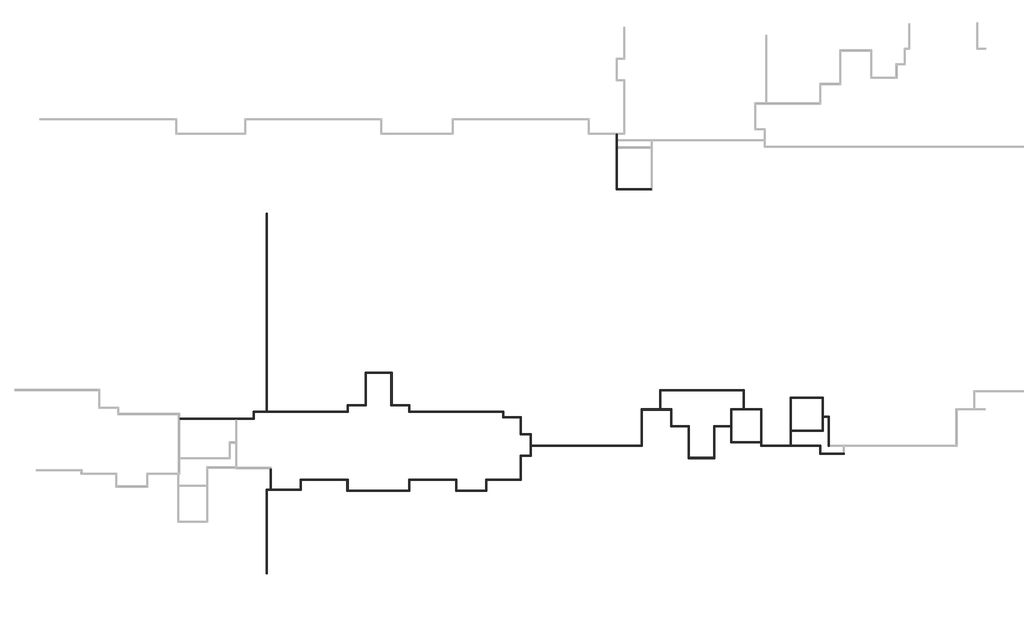
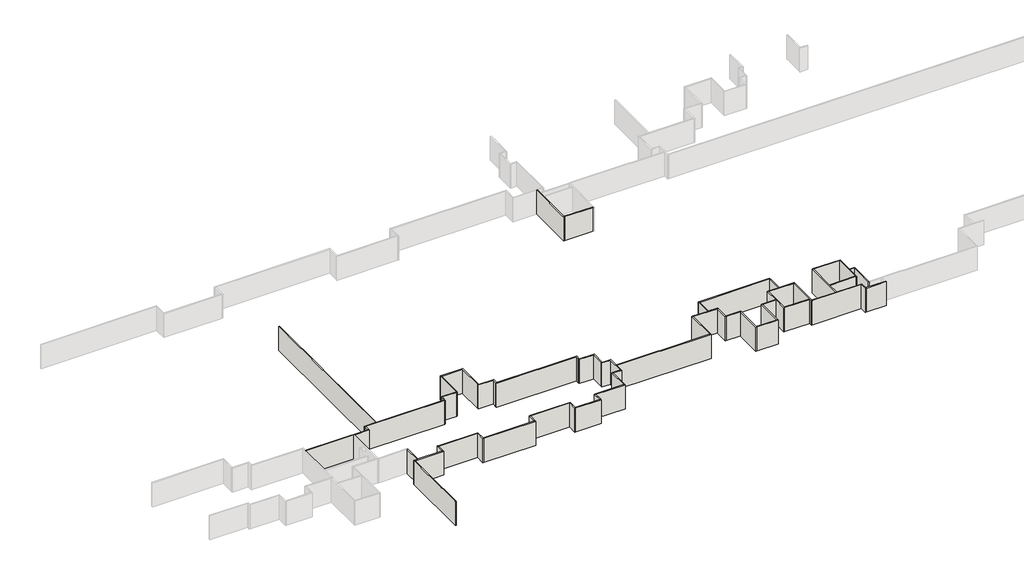
# One storey, part 4 of 8: 59 walls.
"""IFC4 building model written with IfcOpenShell, lengths in millimetres."""

import ifcopenshell
import ifcopenshell.guid

model = None  # the IFC model being written
_history = None  # IfcOwnerHistory: only IFC2X3 demands one
_inside = {}  # id of a spatial element -> (the spatial element, [elements in it])
_under = {}  # id of a project, library or spatial element -> (it, [spatial elements below it])
_declared = {}  # id of a project -> (the project, [libraries it declares])
_typed = {}  # id of a type object -> (the type object, [elements of that type])
_made_of = {}  # id of a material, layer set ... -> (it, [elements and type objects made of it])


def new_model(schema):
    """Start an empty IFC model of exactly this schema.

    Asked for "IFC4X3", IfcOpenShell would pick the latest addendum, in which some entities
    have other attributes; the version numbers below select the first issue.
    IFC2X3 requires an IfcOwnerHistory on every rooted entity: one is made here for all.
    """
    global model, _history
    if schema == "IFC4X3":
        model = ifcopenshell.file(schema_version=(4, 3, 0, 0))
    else:
        model = ifcopenshell.file(schema=schema)
    _inside.clear()
    _under.clear()
    _declared.clear()
    _typed.clear()
    _made_of.clear()
    _history = None
    if model.schema == "IFC2X3":
        org = make("IfcOrganization", Name="unknown")
        user = make(
            "IfcPersonAndOrganization",
            ThePerson=make("IfcPerson", FamilyName="unknown"),
            TheOrganization=org,
        )
        app = make(
            "IfcApplication",
            ApplicationDeveloper=org,
            Version="unknown",
            ApplicationFullName="unknown",
            ApplicationIdentifier="unknown",
        )
        _history = make(
            "IfcOwnerHistory",
            OwningUser=user,
            OwningApplication=app,
            ChangeAction="ADDED",
            CreationDate=0,
        )
    return model


def make(cls, **values):
    """One entity of the class cls with the attributes given. An attribute that is None is left unset."""
    return model.create_entity(
        cls, **{name: value for name, value in values.items() if value is not None}
    )


def rooted(cls, **values):
    """An entity with a GlobalId (a new one), such as an element, a storey or a relation."""
    return make(cls, GlobalId=ifcopenshell.guid.new(), OwnerHistory=_history, **values)


def si_unit(unit_type, name, prefix=None):
    """IfcSIUnit, for example si_unit("LENGTHUNIT", "METRE", prefix="MILLI")."""
    return make("IfcSIUnit", UnitType=unit_type, Prefix=prefix, Name=name)


def assignment(units):
    """IfcUnitAssignment: the units of a project."""
    return None if units is None else make("IfcUnitAssignment", Units=units)


def point(xyz):
    """IfcCartesianPoint."""
    return None if xyz is None else make("IfcCartesianPoint", Coordinates=xyz)


def direction(xyz):
    """IfcDirection."""
    return None if xyz is None else make("IfcDirection", DirectionRatios=xyz)


def frame(location, z_axis=None, x_axis=None):
    """IfcAxis2Placement3D, a coordinate frame: its origin and axes. An axis left out is left unset."""
    return make(
        "IfcAxis2Placement3D",
        Location=point(location),
        Axis=direction(z_axis),
        RefDirection=direction(x_axis),
    )


def origin():
    """The frame at (0, 0, 0) with its axes left unset."""
    return frame((0.0, 0.0, 0.0))


def origin_with_axes():
    """The frame at (0, 0, 0) with the z axis (0, 0, 1) and the x axis (1, 0, 0) written out."""
    return frame((0.0, 0.0, 0.0), z_axis=(0.0, 0.0, 1.0), x_axis=(1.0, 0.0, 0.0))


def place(relative_to, where):
    """IfcLocalPlacement: puts the frame where relative to a parent placement (None: the world)."""
    return make(
        "IfcLocalPlacement", PlacementRelTo=relative_to, RelativePlacement=where
    )


def context(
    kind, dimensions, precision=None, world=None, true_north=None, identifier=None
):
    """IfcGeometricRepresentationContext, for example the 3D "Model" context."""
    return make(
        "IfcGeometricRepresentationContext",
        ContextIdentifier=identifier,
        ContextType=kind,
        CoordinateSpaceDimension=dimensions,
        Precision=precision,
        WorldCoordinateSystem=world,
        TrueNorth=true_north,
    )


def project(units=None, contexts=None):
    """IfcProject with its units and contexts."""
    return rooted(
        "IfcProject",
        Name="project",
        RepresentationContexts=contexts,
        UnitsInContext=assignment(units),
    )


def spatial(cls, under=None, at=None, **own):
    """A site, building, storey or space (cls), placed at a placement, below another one or the project."""
    s = rooted(cls, ObjectPlacement=at, **own)
    if under is not None:
        _under.setdefault(under.id(), (under, []))[1].append(s)
    return s


def polyline(points):
    """IfcPolyline through the points."""
    return make("IfcPolyline", Points=[point(p) for p in points])


def outline(outer, holes=None, kind="AREA"):
    """IfcArbitraryClosedProfileDef: a profile drawn as a closed curve; with holes, ...WithVoids."""
    if holes is None:
        return make("IfcArbitraryClosedProfileDef", ProfileType=kind, OuterCurve=outer)
    return make(
        "IfcArbitraryProfileDefWithVoids",
        ProfileType=kind,
        OuterCurve=outer,
        InnerCurves=holes,
    )


def extrude(swept, where, along, depth):
    """IfcExtrudedAreaSolid: the profile swept, set in the frame where, extruded along a direction by depth."""
    return make(
        "IfcExtrudedAreaSolid",
        SweptArea=swept,
        Position=where,
        ExtrudedDirection=direction(along),
        Depth=depth,
    )


def faces_of(points, faces, orient=None, outer=None):
    """IfcFace entities. A face is a list of loops; a loop is a list of indices into points, from 0.

    orient and outer hold one flag for each loop. By default every Orientation is true, the
    first loop of a face is its IfcFaceOuterBound and the others are IfcFaceBound.
    """
    made = []
    for i, loops in enumerate(faces):
        bounds = []
        for j, loop in enumerate(loops):
            is_outer = j == 0 if outer is None else outer[i][j]
            bounds.append(
                make(
                    "IfcFaceOuterBound" if is_outer else "IfcFaceBound",
                    Bound=make("IfcPolyLoop", Polygon=[points[k] for k in loop]),
                    Orientation=True if orient is None else orient[i][j],
                )
            )
        made.append(make("IfcFace", Bounds=bounds))
    return made


def faceted_brep(points, faces, orient=None, outer=None, voids=None):
    """IfcFacetedBrep: a solid bounded by flat faces; with voids (closed shells), ...WithVoids."""
    shared = [point(p) for p in points]
    hull = make("IfcClosedShell", CfsFaces=faces_of(shared, faces, orient, outer))
    if voids is None:
        return make("IfcFacetedBrep", Outer=hull)
    return make(
        "IfcFacetedBrepWithVoids",
        Outer=hull,
        Voids=[
            make(cls, CfsFaces=faces_of(shared, fs, o, b)) for cls, fs, o, b in voids
        ],
    )


def shape(context_of_items, identifier, shape_type, items):
    """IfcShapeRepresentation: the items that make up one representation, for example the "Body"."""
    return make(
        "IfcShapeRepresentation",
        ContextOfItems=context_of_items,
        RepresentationIdentifier=identifier,
        RepresentationType=shape_type,
        Items=items,
    )


def made_of(thing, what):
    """Note that an element or type object is made of a material, layer set ...; save() writes the relation."""
    if what is not None:
        _made_of.setdefault(what.id(), (what, []))[1].append(thing)
    return thing


def element(
    cls,
    number,
    at=None,
    inside=None,
    cuts=None,
    type_object=None,
    material=None,
    context=None,
    identifier="Body",
    shape_type=None,
    held_by="IfcProductDefinitionShape",
    body=None,
    shapes=None,
    **own,
):
    """One element of the class cls, such as IfcWall. Its Tag is "e" and its number.

    at: its placement. inside: the storey or other place that contains it. cuts: it is an
    opening in that element (IfcRelVoidsElement). A single representation is given by context,
    identifier, shape_type and body (its items); several are given by shapes. held_by: the class
    of the entity that holds the representations. save() writes the other relations.
    """
    e = rooted(cls, Tag="e%d" % number, ObjectPlacement=at, **own)
    if body is not None:
        shapes = [shape(context, identifier, shape_type, body)]
    if shapes is not None:
        e.Representation = make(held_by, Representations=shapes)
    if inside is not None:
        _inside.setdefault(inside.id(), (inside, []))[1].append(e)
    if cuts is not None:
        rooted(
            "IfcRelVoidsElement", RelatingBuildingElement=cuts, RelatedOpeningElement=e
        )
    if type_object is not None:
        _typed.setdefault(type_object.id(), (type_object, []))[1].append(e)
    return made_of(e, material)


def aggregate(whole, parts):
    """IfcRelAggregates: a whole, such as a stair, and the parts it consists of."""
    return rooted("IfcRelAggregates", RelatingObject=whole, RelatedObjects=parts)


def save(model, path):
    """Write the relations noted so far, then the file.

    IfcRelAggregates (storeys below a building ...), IfcRelContainedInSpatialStructure (elements
    in a storey), IfcRelDefinesByType, IfcRelAssociatesMaterial and IfcRelDeclares: one each for
    every whole, place, type object, material and project.
    """
    for whole, parts in _under.values():
        aggregate(whole, parts)
    for where, things in _inside.values():
        rooted(
            "IfcRelContainedInSpatialStructure",
            RelatedElements=things,
            RelatingStructure=where,
        )
    for kind, things in _typed.values():
        rooted("IfcRelDefinesByType", RelatedObjects=things, RelatingType=kind)
    for what, things in _made_of.values():
        rooted("IfcRelAssociatesMaterial", RelatedObjects=things, RelatingMaterial=what)
    for by, libraries in _declared.values():
        rooted("IfcRelDeclares", RelatingContext=by, RelatedDefinitions=libraries)
    model.write(path)


model = new_model("IFC4")

# Units and contexts
model_context = context("Model", 3, world=origin())
ifc_project = project(units=[si_unit("LENGTHUNIT", "METRE", prefix="MILLI")], contexts=[model_context])

# Site, building, storey
site = spatial("IfcSite", under=ifc_project)
building = spatial("IfcBuilding", under=site)
storey = spatial("IfcBuildingStorey", under=building, Name="户型图", Elevation=0.0)

# Walls
placement = place(None, origin())
element("IfcWall", 1, ObjectType="所有墙体", at=placement, inside=storey, context=model_context, shape_type="Brep", body=[
    faceted_brep([(235089.8041277, 123051.6486698, 0.0), (231369.8041277, 123051.6486698, 0.0), (231369.8041277, 123051.6486698, 2700.0), (231369.8041277, 123051.6486698, 3300.0), (235089.8041277, 123051.6486698, 3300.0), (235089.8041277, 123051.6486698, 2700.0), (235089.8041277, 122931.6486698, 0.0), (235089.8041277, 122931.6486698, 2700.0), (235089.8041277, 122931.6486698, 3300.0), (231369.8041277, 122931.6486698, 3300.0), (231369.8041277, 122931.6486698, 0.0)], [[[0, 1, 2, 3, 4, 5]], [[6, 7, 8, 9, 10]], [[1, 0, 6, 10]], [[4, 3, 9, 8]], [[0, 5, 4, 8, 7, 6]], [[3, 2, 1, 10, 9]]]),
])
element("IfcWall", 2, ObjectType="所有墙体", at=placement, inside=storey, context=model_context, shape_type="Brep", body=[
    faceted_brep([(231369.8041277, 122931.6486698, 0.0), (231369.8041277, 123051.6486698, 0.0), (231369.8041277, 127527.7400892, 0.0), (231369.8041277, 127647.7400892, 0.0), (231369.8041277, 128327.7400891, 0.0), (231369.8041277, 128447.7400891, 0.0), (231369.8041277, 129027.5312684, 0.0), (231369.8041277, 129027.5312684, 3300.0), (231369.8041277, 128447.7400891, 3300.0), (231369.8041277, 128327.7400891, 3300.0), (231369.8041277, 127647.7400892, 3300.0), (231369.8041277, 127527.7400892, 3300.0), (231369.8041277, 123192.3894162, 3300.0), (231369.8041277, 123051.6486698, 3300.0), (231369.8041277, 122931.6486698, 3300.0), (231249.8041277, 122931.6486698, 0.0), (231249.8041277, 122931.6486698, 2700.0), (231249.8041277, 122931.6486698, 3300.0), (231249.8041277, 123192.3894162, 3300.0), (231249.8041277, 129027.5312684, 3300.0), (231249.8041277, 129027.5312684, 0.0)], [[[0, 1, 2, 3, 4, 5, 6, 7, 8, 9, 10, 11, 12, 13, 14]], [[15, 16, 17, 18, 19, 20]], [[6, 5, 4, 3, 2, 1, 0, 15, 20]], [[14, 13, 12, 11, 10, 9, 8, 7, 19, 18, 17]], [[0, 14, 17, 16, 15]], [[7, 6, 20, 19]]]),
])
element("IfcWall", 3, ObjectType="所有墙体", at=placement, inside=storey, context=model_context, shape_type="Brep", body=[
    faceted_brep([(192640.3009401, 120342.1448334, 0.0), (192640.3009401, 98502.1085876, 0.0), (192640.3009401, 98502.1085876, 3300.0), (192640.3009401, 104192.1448334, 3300.0), (192640.3009401, 110342.1448334, 3300.0), (192640.3009401, 110492.1448334, 3300.0), (192640.3009401, 115192.1448334, 3300.0), (192640.3009401, 115492.1448334, 3300.0), (192640.3009401, 120192.1448334, 3300.0), (192640.3009401, 120342.1448334, 3300.0), (192760.3009401, 120342.1448334, 0.0), (192760.3009401, 120342.1448334, 3300.0), (192760.3009401, 120192.1448334, 3300.0), (192760.3009401, 115342.1448334, 3300.0), (192760.3009401, 115192.1448334, 3300.0), (192760.3009401, 110492.1448334, 3300.0), (192760.3009401, 110342.1448334, 3300.0), (192760.3009401, 104192.1448334, 3300.0), (192760.3009401, 98502.1084133, 3300.0), (192760.3009401, 98502.1084133, 0.0)], [[[0, 1, 2, 3, 4, 5, 6, 7, 8, 9]], [[10, 11, 12, 13, 14, 15, 16, 17, 18, 19]], [[1, 0, 10, 19]], [[9, 8, 7, 6, 5, 4, 3, 2, 18, 17, 16, 15, 14, 13, 12, 11]], [[0, 9, 11, 10]], [[2, 1, 19, 18]]]),
])
element("IfcWall", 4, ObjectType="所有墙体", at=placement, inside=storey, context=model_context, shape_type="Brep", body=[
    faceted_brep([(201562.0411038, 98502.095626, 0.0), (192760.3009401, 98502.1084133, 0.0), (192640.3009401, 98502.1085876, 0.0), (191179.3333405, 98502.1107101, 0.0), (191179.3333405, 98502.1107101, 3300.0), (192640.3009401, 98502.1085876, 3300.0), (192760.3009401, 98502.1084133, 3300.0), (201562.0411038, 98502.095626, 3300.0), (201562.0411038, 98382.095626, 0.0), (201562.0411038, 98382.095626, 3300.0), (191299.3333405, 98382.1105358, 3300.0), (191179.3333405, 98382.1107101, 3300.0), (191179.3333405, 98382.1107101, 0.0), (191299.3333405, 98382.1105358, 0.0)], [[[0, 1, 2, 3, 4, 5, 6, 7]], [[8, 9, 10, 11, 12, 13]], [[3, 2, 1, 0, 8, 13, 12]], [[7, 6, 5, 4, 11, 10, 9]], [[4, 3, 12, 11]], [[0, 7, 9, 8]]]),
])
element("IfcWall", 5, ObjectType="所有墙体", at=placement, inside=storey, context=model_context, shape_type="SweptSolid", body=[
    extrude(outline(polyline([(191179.3333405, 97732.4890874), (191179.3333405, 98382.1107101), (191299.3333405, 98382.1105358), (191299.3333405, 97732.4890874), (191179.3333405, 97732.4890874)])), origin_with_axes(), (0.0, 0.0, 1.0), 3300.0),
])
element("IfcWall", 6, ObjectType="所有墙体", at=placement, inside=storey, context=model_context, shape_type="SweptSolid", body=[
    extrude(outline(polyline([(193080.9640604, 89902.0416967), (193080.9640604, 92173.7889647), (193200.9640604, 92173.7889647), (193200.9640604, 89902.0416967), (193080.9640604, 89902.0416967)])), origin_with_axes(), (0.0, 0.0, 1.0), 3300.0),
])
element("IfcWall", 7, ObjectType="所有墙体", at=placement, inside=storey, context=model_context, shape_type="Brep", body=[
    faceted_brep([(196500.9640604, 89902.0416967, 0.0), (196380.9640604, 89902.0416967, 0.0), (193200.9640604, 89902.0416967, 0.0), (193080.9640604, 89902.0416967, 0.0), (192640.3009401, 89902.0416967, 0.0), (192640.3009401, 89902.0416967, 3300.0), (193080.9640604, 89902.0416967, 3300.0), (193200.9640604, 89902.0416967, 3300.0), (196380.9640604, 89902.0416967, 3300.0), (196500.9640604, 89902.0416967, 3300.0), (196500.9640604, 89782.0416967, 0.0), (196500.9640604, 89782.0416967, 3300.0), (192760.3009401, 89782.0416967, 3300.0), (192640.3009401, 89782.0416967, 3300.0), (192640.3009401, 89782.0416967, 0.0), (192760.3009401, 89782.0416967, 0.0)], [[[0, 1, 2, 3, 4, 5, 6, 7, 8, 9]], [[10, 11, 12, 13, 14, 15]], [[4, 3, 2, 1, 0, 10, 15, 14]], [[9, 8, 7, 6, 5, 13, 12, 11]], [[5, 4, 14, 13]], [[0, 9, 11, 10]]]),
])
element("IfcWall", 8, ObjectType="所有墙体", at=placement, inside=storey, context=model_context, shape_type="Brep", body=[
    faceted_brep([(192640.3009401, 89782.0416967, 0.0), (192640.3009401, 80542.0416967, 0.0), (192640.3009401, 80542.0416967, 2700.0), (192640.3009401, 80542.0416967, 3300.0), (192640.3009401, 80676.6002718, 3300.0), (192640.3009401, 86381.1826239, 3300.0), (192640.3009401, 86681.1826239, 3300.0), (192640.3009401, 89782.0416967, 3300.0), (192760.3009401, 89782.0416967, 0.0), (192760.3009401, 89782.0416967, 3300.0), (192760.3009401, 86681.1826239, 3300.0), (192760.3009401, 86381.1826239, 3300.0), (192760.3009401, 80542.0416967, 3300.0), (192760.3009401, 80542.0416967, 0.0), (192711.3752265, 80542.0416967, 3300.0)], [[[0, 1, 2, 3, 4, 5, 6, 7]], [[8, 9, 10, 11, 12, 13]], [[1, 0, 8, 13]], [[3, 2, 1, 13, 12, 14]], [[7, 6, 5, 4, 3, 14, 12, 11, 10, 9]], [[0, 7, 9, 8]]]),
])
element("IfcWall", 9, ObjectType="所有墙体", at=placement, inside=storey, context=model_context, shape_type="Brep", body=[
    faceted_brep([(196500.9640604, 89902.0416967, 0.0), (196500.9640604, 90882.0439942, 0.0), (196500.9640604, 91002.0439942, 0.0), (196500.9640604, 91002.0439942, 3300.0), (196500.9640604, 90882.0439942, 3300.0), (196500.9640604, 89902.0416967, 3300.0), (196380.9640604, 89902.0416967, 0.0), (196380.9640604, 89902.0416967, 3300.0), (196380.9640604, 91002.0439942, 3300.0), (196380.9640604, 91002.0439942, 0.0)], [[[0, 1, 2, 3, 4, 5]], [[6, 7, 8, 9]], [[2, 1, 0, 6, 9]], [[5, 4, 3, 8, 7]], [[0, 5, 7, 6]], [[3, 2, 9, 8]]]),
])
element("IfcWall", 10, ObjectType="所有墙体", at=placement, inside=storey, context=model_context, shape_type="Brep", body=[
    faceted_brep([(196500.9640604, 90882.0439942, 0.0), (201529.2467743, 90882.0439942, 0.0), (201649.2467743, 90882.0439942, 0.0), (201649.2467743, 90882.0439942, 3300.0), (201529.2467743, 90882.0439942, 3300.0), (196500.9640604, 90882.0439942, 3300.0), (196500.9640604, 91002.0439942, 0.0), (196500.9640604, 91002.0439942, 3300.0), (201649.2467743, 91002.0439942, 3300.0), (201649.2467743, 91002.0439942, 0.0)], [[[0, 1, 2, 3, 4, 5]], [[6, 7, 8, 9]], [[2, 1, 0, 6, 9]], [[5, 4, 3, 8, 7]], [[0, 5, 7, 6]], [[3, 2, 9, 8]]]),
])
element("IfcWall", 11, ObjectType="所有墙体", at=placement, inside=storey, context=model_context, shape_type="Brep", body=[
    faceted_brep([(201529.2467743, 90882.0439942, 0.0), (201529.2467743, 89682.0439941, 0.0), (201529.2467743, 89682.0439941, 3300.0), (201529.2467743, 90882.0439942, 3300.0), (201649.2467743, 90882.0439942, 0.0), (201649.2467743, 90882.0439942, 3300.0), (201649.2467743, 89802.0439941, 3300.0), (201649.2467743, 89682.0439941, 3300.0), (201649.2467743, 89682.0439941, 0.0), (201649.2467743, 89802.0439941, 0.0), (201532.0411038, 89682.0439941, 3300.0)], [[[0, 1, 2, 3]], [[4, 5, 6, 7, 8, 9]], [[1, 0, 4, 9, 8]], [[3, 2, 10, 7, 6, 5]], [[0, 3, 5, 4]], [[2, 1, 8, 7, 10]]]),
])
element("IfcWall", 12, ObjectType="所有墙体", at=placement, inside=storey, context=model_context, shape_type="Brep", body=[
    faceted_brep([(201649.2467743, 89682.0439941, 0.0), (208449.2467743, 89682.0439941, 0.0), (208449.2467743, 89682.0439941, 3300.0), (201649.2467743, 89682.0439941, 3300.0), (201649.2467743, 89802.0439941, 0.0), (201649.2467743, 89802.0439941, 3300.0), (208329.2467743, 89802.0439941, 3300.0), (208449.2467743, 89802.0439941, 3300.0), (208449.2467743, 89802.0439941, 0.0), (208329.2467743, 89802.0439941, 0.0)], [[[0, 1, 2, 3]], [[4, 5, 6, 7, 8, 9]], [[1, 0, 4, 9, 8]], [[3, 2, 7, 6, 5]], [[0, 3, 5, 4]], [[2, 1, 8, 7]]]),
])
element("IfcWall", 13, ObjectType="所有墙体", at=placement, inside=storey, context=model_context, shape_type="Brep", body=[
    faceted_brep([(208449.2467743, 89802.0439941, 0.0), (208449.2467743, 90882.0439942, 0.0), (208449.2467743, 91002.0439942, 0.0), (208449.2467743, 91002.0439942, 3300.0), (208449.2467743, 90882.0439942, 3300.0), (208449.2467743, 89802.0439941, 3300.0), (208329.2467743, 89802.0439941, 0.0), (208329.2467743, 89802.0439941, 3300.0), (208329.2467743, 91002.0439942, 3300.0), (208329.2467743, 91002.0439942, 0.0)], [[[0, 1, 2, 3, 4, 5]], [[6, 7, 8, 9]], [[2, 1, 0, 6, 9]], [[5, 4, 3, 8, 7]], [[0, 5, 7, 6]], [[3, 2, 9, 8]]]),
])
element("IfcWall", 14, ObjectType="所有墙体", at=placement, inside=storey, context=model_context, shape_type="Brep", body=[
    faceted_brep([(208449.2467743, 90882.0439942, 0.0), (213529.2467743, 90882.0439942, 0.0), (213649.2467743, 90882.0439942, 0.0), (213649.2467743, 90882.0439942, 3300.0), (213529.2467743, 90882.0439942, 3300.0), (208449.2467743, 90882.0439942, 3300.0), (208449.2467743, 91002.0439942, 0.0), (208449.2467743, 91002.0439942, 3300.0), (213649.2467743, 91002.0439942, 3300.0), (213649.2467743, 91002.0439942, 0.0)], [[[0, 1, 2, 3, 4, 5]], [[6, 7, 8, 9]], [[2, 1, 0, 6, 9]], [[5, 4, 3, 8, 7]], [[0, 5, 7, 6]], [[3, 2, 9, 8]]]),
])
element("IfcWall", 15, ObjectType="所有墙体", at=placement, inside=storey, context=model_context, shape_type="Brep", body=[
    faceted_brep([(213529.2467743, 90882.0439942, 0.0), (213529.2467743, 89682.0439941, 0.0), (213529.2467743, 89682.0439941, 3300.0), (213529.2467743, 90882.0439942, 3300.0), (213649.2467743, 90882.0439942, 0.0), (213649.2467743, 90882.0439942, 3300.0), (213649.2467743, 89802.0439941, 3300.0), (213649.2467743, 89682.0439941, 3300.0), (213649.2467743, 89682.0439941, 0.0), (213649.2467743, 89802.0439941, 0.0), (213543.6038603, 89682.0439941, 3300.0)], [[[0, 1, 2, 3]], [[4, 5, 6, 7, 8, 9]], [[1, 0, 4, 9, 8]], [[3, 2, 10, 7, 6, 5]], [[0, 3, 5, 4]], [[2, 1, 8, 7, 10]]]),
])
element("IfcWall", 16, ObjectType="所有墙体", at=placement, inside=storey, context=model_context, shape_type="Brep", body=[
    faceted_brep([(213649.2467743, 89682.0439941, 0.0), (216949.2467743, 89682.0439941, 0.0), (216949.2467743, 89682.0439941, 3300.0), (213649.2467743, 89682.0439941, 3300.0), (213649.2467743, 89802.0439941, 0.0), (213649.2467743, 89802.0439941, 3300.0), (216829.2467743, 89802.0439941, 3300.0), (216949.2467743, 89802.0439941, 3300.0), (216949.2467743, 89802.0439941, 0.0), (216829.2467743, 89802.0439941, 0.0)], [[[0, 1, 2, 3]], [[4, 5, 6, 7, 8, 9]], [[1, 0, 4, 9, 8]], [[3, 2, 7, 6, 5]], [[0, 3, 5, 4]], [[2, 1, 8, 7]]]),
])
element("IfcWall", 17, ObjectType="所有墙体", at=placement, inside=storey, context=model_context, shape_type="Brep", body=[
    faceted_brep([(216949.2467743, 89802.0439941, 0.0), (216949.2467743, 90882.0439942, 0.0), (216949.2467743, 91002.0439942, 0.0), (216949.2467743, 91002.0439942, 3300.0), (216949.2467743, 90882.0439942, 3300.0), (216949.2467743, 89802.0439941, 3300.0), (216829.2467743, 89802.0439941, 0.0), (216829.2467743, 89802.0439941, 3300.0), (216829.2467743, 91002.0439942, 3300.0), (216829.2467743, 91002.0439942, 0.0)], [[[0, 1, 2, 3, 4, 5]], [[6, 7, 8, 9]], [[2, 1, 0, 6, 9]], [[5, 4, 3, 8, 7]], [[0, 5, 7, 6]], [[3, 2, 9, 8]]]),
])
element("IfcWall", 18, ObjectType="所有墙体", at=placement, inside=storey, context=model_context, shape_type="Brep", body=[
    faceted_brep([(216949.2467743, 90882.0439942, 0.0), (220749.247895, 90882.0439942, 0.0), (220749.247895, 90882.0439942, 3300.0), (216949.2467743, 90882.0439942, 3300.0), (216949.2467743, 91002.0439942, 0.0), (216949.2467743, 91002.0439942, 3300.0), (220629.247895, 91002.0439942, 3300.0), (220749.247895, 91002.0439942, 3300.0), (220749.247895, 91002.0439942, 0.0), (220629.247895, 91002.0439942, 0.0)], [[[0, 1, 2, 3]], [[4, 5, 6, 7, 8, 9]], [[1, 0, 4, 9, 8]], [[3, 2, 7, 6, 5]], [[0, 3, 5, 4]], [[2, 1, 8, 7]]]),
])
element("IfcWall", 19, ObjectType="所有墙体", at=placement, inside=storey, context=model_context, shape_type="Brep", body=[
    faceted_brep([(220749.247895, 91002.0439942, 0.0), (220749.247895, 93532.0853498, 0.0), (220749.247895, 93652.0853498, 0.0), (220749.247895, 93652.0853498, 3300.0), (220749.247895, 93532.0853498, 3300.0), (220749.247895, 91002.0439942, 3300.0), (220629.247895, 91002.0439942, 0.0), (220629.247895, 91002.0439942, 3300.0), (220629.247895, 93652.0853498, 3300.0), (220629.247895, 93652.0853498, 0.0)], [[[0, 1, 2, 3, 4, 5]], [[6, 7, 8, 9]], [[2, 1, 0, 6, 9]], [[5, 4, 3, 8, 7]], [[0, 5, 7, 6]], [[3, 2, 9, 8]]]),
])
element("IfcWall", 20, ObjectType="所有墙体", at=placement, inside=storey, context=model_context, shape_type="Brep", body=[
    faceted_brep([(220749.247895, 93532.0853498, 0.0), (221849.0862212, 93532.0853498, 0.0), (221849.0862212, 93532.0853498, 3300.0), (220749.247895, 93532.0853498, 3300.0), (220749.247895, 93652.0853498, 0.0), (220749.247895, 93652.0853498, 3300.0), (221729.0862212, 93652.0853498, 3300.0), (221849.0862212, 93652.0853498, 3300.0), (221849.0862212, 93652.0853498, 0.0), (221729.0862212, 93652.0853498, 0.0)], [[[0, 1, 2, 3]], [[4, 5, 6, 7, 8, 9]], [[1, 0, 4, 9, 8]], [[3, 2, 7, 6, 5]], [[0, 3, 5, 4]], [[2, 1, 8, 7]]]),
])
element("IfcWall", 21, ObjectType="所有墙体", at=placement, inside=storey, context=model_context, shape_type="Brep", body=[
    faceted_brep([(221849.0862212, 93652.0853498, 0.0), (221849.0862212, 94629.6848758, 0.0), (221849.0862212, 94749.6848758, 0.0), (221849.0862212, 96002.0586165, 0.0), (221849.0862212, 96002.0586165, 3300.0), (221849.0862212, 94749.6848758, 3300.0), (221849.0862212, 94629.6848758, 3300.0), (221849.0862212, 93652.0853498, 3300.0), (221729.0862212, 93652.0853498, 0.0), (221729.0862212, 93652.0853498, 3300.0), (221729.0862212, 95882.0586165, 3300.0), (221729.0862212, 96002.0586165, 3300.0), (221729.0862212, 96002.0586165, 0.0), (221729.0862212, 95882.0586165, 0.0)], [[[0, 1, 2, 3, 4, 5, 6, 7]], [[8, 9, 10, 11, 12, 13]], [[3, 2, 1, 0, 8, 13, 12]], [[7, 6, 5, 4, 11, 10, 9]], [[0, 7, 9, 8]], [[4, 3, 12, 11]]]),
])
element("IfcWall", 22, ObjectType="所有墙体", at=placement, inside=storey, context=model_context, shape_type="Brep", body=[
    faceted_brep([(221729.0862212, 96002.0586165, 0.0), (220749.247895, 96002.0586165, 0.0), (220629.247895, 96002.0586165, 0.0), (220629.247895, 96002.0586165, 3300.0), (220749.247895, 96002.0586165, 3300.0), (221729.0862212, 96002.0586165, 3300.0), (221729.0862212, 95882.0586165, 0.0), (221729.0862212, 95882.0586165, 3300.0), (220629.247895, 95882.0586165, 3300.0), (220629.247895, 95882.0586165, 0.0)], [[[0, 1, 2, 3, 4, 5]], [[6, 7, 8, 9]], [[2, 1, 0, 6, 9]], [[5, 4, 3, 8, 7]], [[0, 5, 7, 6]], [[3, 2, 9, 8]]]),
])
element("IfcWall", 23, ObjectType="所有墙体", at=placement, inside=storey, context=model_context, shape_type="Brep", body=[
    faceted_brep([(220749.247895, 96002.0586165, 0.0), (220749.247895, 97885.8817439, 0.0), (220749.247895, 97885.8817439, 3300.0), (220749.247895, 96002.0586165, 3300.0), (220629.247895, 96002.0586165, 0.0), (220629.247895, 96002.0586165, 3300.0), (220629.247895, 97765.8817439, 3300.0), (220629.247895, 97885.8817439, 3300.0), (220629.247895, 97885.8817439, 0.0), (220629.247895, 97765.8817439, 0.0)], [[[0, 1, 2, 3]], [[4, 5, 6, 7, 8, 9]], [[1, 0, 4, 9, 8]], [[3, 2, 7, 6, 5]], [[0, 3, 5, 4]], [[2, 1, 8, 7]]]),
])
element("IfcWall", 24, ObjectType="所有墙体", at=placement, inside=storey, context=model_context, shape_type="Brep", body=[
    faceted_brep([(220629.247895, 97885.8817439, 0.0), (218849.3333405, 97885.8817439, 0.0), (218729.3333405, 97885.8817439, 0.0), (218729.3333405, 97885.8817439, 3300.0), (218849.3333405, 97885.8817439, 3300.0), (220629.247895, 97885.8817439, 3300.0), (220629.247895, 97765.8817439, 0.0), (220629.247895, 97765.8817439, 3300.0), (218729.3333405, 97765.8817439, 3300.0), (218729.3333405, 97765.8817439, 0.0)], [[[0, 1, 2, 3, 4, 5]], [[6, 7, 8, 9]], [[2, 1, 0, 6, 9]], [[5, 4, 3, 8, 7]], [[0, 5, 7, 6]], [[3, 2, 9, 8]]]),
])
element("IfcWall", 25, ObjectType="所有墙体", at=placement, inside=storey, context=model_context, shape_type="Brep", body=[
    faceted_brep([(218849.3333405, 97885.8817439, 0.0), (218849.3333405, 98502.0955388, 0.0), (218849.3333405, 98502.0955388, 3300.0), (218849.3333405, 97885.8817439, 3300.0), (218729.3333405, 97885.8817439, 0.0), (218729.3333405, 97885.8817439, 3300.0), (218729.3333405, 98382.0955388, 3300.0), (218729.3333405, 98502.0955388, 3300.0), (218729.3333405, 98502.0955388, 0.0), (218729.3333405, 98382.0955388, 0.0)], [[[0, 1, 2, 3]], [[4, 5, 6, 7, 8, 9]], [[1, 0, 4, 9, 8]], [[3, 2, 7, 6, 5]], [[0, 3, 5, 4]], [[2, 1, 8, 7]]]),
])
element("IfcWall", 26, ObjectType="所有墙体", at=placement, inside=storey, context=model_context, shape_type="Brep", body=[
    faceted_brep([(218729.3333405, 98502.0955388, 0.0), (208449.2467743, 98502.0955388, 0.0), (208329.2467743, 98502.0955388, 0.0), (208329.2467743, 98502.0955388, 3300.0), (208449.2467743, 98502.0955388, 3300.0), (213550.3009384, 98502.0955388, 3300.0), (213850.3009384, 98502.0955388, 3300.0), (218729.3333405, 98502.0955388, 3300.0), (218729.3333405, 98382.0955388, 0.0), (218729.3333405, 98382.0955388, 3300.0), (213850.3009384, 98382.0955388, 3300.0), (213550.3009384, 98382.0955388, 3300.0), (208329.2467743, 98382.0955388, 3300.0), (208329.2467743, 98382.0955388, 0.0)], [[[0, 1, 2, 3, 4, 5, 6, 7]], [[8, 9, 10, 11, 12, 13]], [[2, 1, 0, 8, 13]], [[7, 6, 5, 4, 3, 12, 11, 10, 9]], [[0, 7, 9, 8]], [[3, 2, 13, 12]]]),
])
element("IfcWall", 27, ObjectType="所有墙体", at=placement, inside=storey, context=model_context, shape_type="Brep", body=[
    faceted_brep([(208449.2467743, 98502.0955388, 0.0), (208449.2467743, 99202.0955388, 0.0), (208449.2467743, 99202.0955388, 2700.0), (208449.2467743, 99202.0955388, 3300.0), (208449.2467743, 99082.0955388, 3300.0), (208449.2467743, 98502.0955388, 3300.0), (208329.2467743, 98502.0955388, 0.0), (208329.2467743, 98502.0955388, 3300.0), (208329.2467743, 99082.0955388, 3300.0), (208329.2467743, 99202.0955388, 3300.0), (208329.2467743, 99202.0955388, 0.0), (208329.2467743, 99082.0955388, 0.0)], [[[0, 1, 2, 3, 4, 5]], [[6, 7, 8, 9, 10, 11]], [[1, 0, 6, 11, 10]], [[5, 4, 3, 9, 8, 7]], [[0, 5, 7, 6]], [[3, 2, 1, 10, 9]]]),
])
element("IfcWall", 28, ObjectType="所有墙体", at=placement, inside=storey, context=model_context, shape_type="Brep", body=[
    faceted_brep([(208329.2467743, 99202.0955388, 0.0), (206499.3333102, 99202.0955388, 0.0), (206379.3333102, 99202.0955388, 0.0), (206379.3333102, 99202.0955388, 3300.0), (206499.3333102, 99202.0955388, 3300.0), (208329.2467743, 99202.0955388, 3300.0), (208329.2467743, 99082.0955388, 0.0), (208329.2467743, 99082.0955388, 3300.0), (206379.3333102, 99082.0955388, 3300.0), (206379.3333102, 99082.0955388, 0.0)], [[[0, 1, 2, 3, 4, 5]], [[6, 7, 8, 9]], [[2, 1, 0, 6, 9]], [[5, 4, 3, 8, 7]], [[0, 5, 7, 6]], [[3, 2, 9, 8]]]),
])
element("IfcWall", 29, ObjectType="所有墙体", at=placement, inside=storey, context=model_context, shape_type="Brep", body=[
    faceted_brep([(206499.3333102, 99202.0955388, 0.0), (206499.3333102, 102802.0439942, 0.0), (206499.3333102, 102802.0439942, 3300.0), (206499.3333102, 99202.0955388, 3300.0), (206379.3333102, 99202.0955388, 0.0), (206379.3333102, 99202.0955388, 3300.0), (206379.3333102, 102682.0439942, 3300.0), (206379.3333102, 102802.0439942, 3300.0), (206379.3333102, 102802.0439942, 0.0), (206379.3333102, 102682.0439942, 0.0)], [[[0, 1, 2, 3]], [[4, 5, 6, 7, 8, 9]], [[1, 0, 4, 9, 8]], [[3, 2, 7, 6, 5]], [[0, 3, 5, 4]], [[2, 1, 8, 7]]]),
])
element("IfcWall", 30, ObjectType="所有墙体", at=placement, inside=storey, context=model_context, shape_type="Brep", body=[
    faceted_brep([(206379.3333102, 102802.0439942, 0.0), (203529.3322199, 102802.0439942, 0.0), (203529.3322199, 102802.0439942, 3300.0), (206379.3333102, 102802.0439942, 3300.0), (206379.3333102, 102682.0439942, 0.0), (206379.3333102, 102682.0439942, 3300.0), (203649.3322199, 102682.0439942, 3300.0), (203529.3322199, 102682.0439942, 3300.0), (203529.3322199, 102682.0439942, 0.0), (203649.3322199, 102682.0439942, 0.0)], [[[0, 1, 2, 3]], [[4, 5, 6, 7, 8, 9]], [[1, 0, 4, 9, 8]], [[3, 2, 7, 6, 5]], [[0, 3, 5, 4]], [[2, 1, 8, 7]]]),
])
element("IfcWall", 31, ObjectType="所有墙体", at=placement, inside=storey, context=model_context, shape_type="Brep", body=[
    faceted_brep([(203529.3322199, 102682.0439942, 0.0), (203529.3322199, 99202.0955388, 0.0), (203529.3322199, 99082.0955388, 0.0), (203529.3322199, 99082.0955388, 3300.0), (203529.3322199, 99202.0955388, 3300.0), (203529.3322199, 102682.0439942, 3300.0), (203649.3322199, 102682.0439942, 0.0), (203649.3322199, 102682.0439942, 3300.0), (203649.3322199, 99082.0955388, 3300.0), (203649.3322199, 99082.0955388, 0.0)], [[[0, 1, 2, 3, 4, 5]], [[6, 7, 8, 9]], [[2, 1, 0, 6, 9]], [[5, 4, 3, 8, 7]], [[0, 5, 7, 6]], [[3, 2, 9, 8]]]),
])
element("IfcWall", 32, ObjectType="所有墙体", at=placement, inside=storey, context=model_context, shape_type="Brep", body=[
    faceted_brep([(203529.3322199, 99202.0955388, 0.0), (201562.0411038, 99202.0955388, 0.0), (201562.0411038, 99202.0955388, 3300.0), (203529.3322199, 99202.0955388, 3300.0), (203529.3322199, 99082.0955388, 0.0), (203529.3322199, 99082.0955388, 3300.0), (201682.0411038, 99082.0955388, 3300.0), (201562.0411038, 99082.0955388, 3300.0), (201562.0411038, 99082.0955388, 0.0), (201682.0411038, 99082.0955388, 0.0)], [[[0, 1, 2, 3]], [[4, 5, 6, 7, 8, 9]], [[1, 0, 4, 9, 8]], [[3, 2, 7, 6, 5]], [[0, 3, 5, 4]], [[2, 1, 8, 7]]]),
])
element("IfcWall", 33, ObjectType="所有墙体", at=placement, inside=storey, context=model_context, shape_type="Brep", body=[
    faceted_brep([(201562.0411038, 99082.0955388, 0.0), (201562.0411038, 98502.095626, 0.0), (201562.0411038, 98382.095626, 0.0), (201562.0411038, 98382.095626, 3300.0), (201562.0411038, 98502.095626, 3300.0), (201562.0411038, 99082.0955388, 3300.0), (201682.0411038, 99082.0955388, 0.0), (201682.0411038, 99082.0955388, 3300.0), (201682.0411038, 98382.0954516, 3300.0), (201682.0411038, 98382.0954516, 0.0)], [[[0, 1, 2, 3, 4, 5]], [[6, 7, 8, 9]], [[2, 1, 0, 6, 9]], [[5, 4, 3, 8, 7]], [[0, 5, 7, 6]], [[3, 2, 9, 8]]]),
])
element("IfcWall", 34, ObjectType="所有墙体", at=placement, inside=storey, context=model_context, shape_type="Brep", body=[
    faceted_brep([(183060.4077201, 97612.4890874, 0.0), (189279.4180303, 97612.4890874, 0.0), (189399.4180303, 97612.4890874, 0.0), (191300.4077201, 97612.4890874, 0.0), (191300.4077201, 97612.4890874, 3300.0), (189399.4180303, 97612.4890874, 3300.0), (189279.4180303, 97612.4890874, 3300.0), (183060.4077201, 97612.4890874, 3300.0), (183060.4077201, 97732.4890874, 0.0), (183060.4077201, 97732.4890874, 3300.0), (191179.3333405, 97732.4890874, 3300.0), (191299.3333405, 97732.4890874, 3300.0), (191300.4077201, 97732.4890874, 3300.0), (191300.4077201, 97732.4890874, 0.0), (191299.3333405, 97732.4890874, 0.0), (191179.3333405, 97732.4890874, 0.0)], [[[0, 1, 2, 3, 4, 5, 6, 7]], [[8, 9, 10, 11, 12, 13, 14, 15]], [[3, 2, 1, 0, 8, 15, 14, 13]], [[4, 3, 13, 12]], [[7, 6, 5, 4, 12, 11, 10, 9]], [[0, 7, 9, 8]]]),
])
element("IfcWall", 35, ObjectType="所有墙体", at=placement, inside=storey, context=model_context, shape_type="Brep", body=[
    faceted_brep([(221849.0862212, 94629.6848758, 0.0), (234125.5103964, 94629.6848758, 0.0), (234125.5103964, 94629.6848758, 3300.0), (227628.8819762, 94629.6848758, 3300.0), (227328.1494068, 94629.6848758, 3300.0), (221849.0862212, 94629.6848758, 3300.0), (221849.0862212, 94749.6848758, 0.0), (221849.0862212, 94749.6848758, 3300.0), (227319.7581894, 94749.6848758, 3300.0), (227620.4907588, 94749.6848758, 3300.0), (234005.5103964, 94749.6848758, 3300.0), (234125.5103964, 94749.6848758, 3300.0), (234125.5103964, 94749.6848758, 0.0), (234005.5103964, 94749.6848758, 0.0)], [[[0, 1, 2, 3, 4, 5]], [[6, 7, 8, 9, 10, 11, 12, 13]], [[1, 0, 6, 13, 12]], [[5, 4, 3, 2, 11, 10, 9, 8, 7]], [[0, 5, 7, 6]], [[2, 1, 12, 11]]]),
])
element("IfcWall", 36, ObjectType="所有墙体", at=placement, inside=storey, context=model_context, shape_type="Brep", body=[
    faceted_brep([(234125.5103964, 94749.6848758, 0.0), (234125.5103964, 98630.1217457, 0.0), (234125.5103964, 98750.1217457, 0.0), (234125.5103964, 98750.1217457, 3300.0), (234125.5103964, 98630.1217457, 3300.0), (234125.5103964, 94749.6848758, 3300.0), (234005.5103964, 94749.6848758, 0.0), (234005.5103964, 94749.6848758, 3300.0), (234005.5103964, 98750.1217457, 3300.0), (234005.5103964, 98750.1217457, 0.0)], [[[0, 1, 2, 3, 4, 5]], [[6, 7, 8, 9]], [[2, 1, 0, 6, 9]], [[5, 4, 3, 8, 7]], [[0, 5, 7, 6]], [[3, 2, 9, 8]]]),
])
element("IfcWall", 37, ObjectType="所有墙体", at=placement, inside=storey, context=model_context, shape_type="Brep", body=[
    faceted_brep([(234125.5103964, 98630.1217457, 0.0), (237239.6710131, 98630.1217457, 0.0), (237359.6710131, 98630.1217457, 0.0), (237359.6710131, 98630.1217457, 3300.0), (237239.6710131, 98630.1217457, 3300.0), (234125.5103964, 98630.1217457, 3300.0), (234125.5103964, 98750.1217457, 0.0), (234125.5103964, 98750.1217457, 3300.0), (236039.6710138, 98750.1217457, 3300.0), (236159.6710138, 98750.1217457, 3300.0), (237359.6710131, 98750.1217457, 3300.0), (237359.6710131, 98750.1217457, 0.0), (236159.6710138, 98750.1217457, 0.0), (236039.6710138, 98750.1217457, 0.0)], [[[0, 1, 2, 3, 4, 5]], [[6, 7, 8, 9, 10, 11, 12, 13]], [[2, 1, 0, 6, 13, 12, 11]], [[5, 4, 3, 10, 9, 8, 7]], [[0, 5, 7, 6]], [[3, 2, 11, 10]]]),
])
element("IfcWall", 38, ObjectType="所有墙体", at=placement, inside=storey, context=model_context, shape_type="Brep", body=[
    faceted_brep([(237239.6710131, 98630.1217457, 0.0), (237239.6710131, 96780.8975721, 0.0), (237239.6710131, 96780.8975721, 3300.0), (237239.6710131, 98630.1217457, 3300.0), (237359.6710131, 98630.1217457, 0.0), (237359.6710131, 98630.1217457, 3300.0), (237359.6710131, 96900.8975721, 3300.0), (237359.6710131, 96780.8975721, 3300.0), (237359.6710131, 96780.8975721, 0.0), (237359.6710131, 96900.8975721, 0.0)], [[[0, 1, 2, 3]], [[4, 5, 6, 7, 8, 9]], [[1, 0, 4, 9, 8]], [[3, 2, 7, 6, 5]], [[0, 3, 5, 4]], [[2, 1, 8, 7]]]),
])
element("IfcWall", 39, ObjectType="所有墙体", at=placement, inside=storey, context=model_context, shape_type="Brep", body=[
    faceted_brep([(237359.6710131, 96780.8975721, 0.0), (239189.671013, 96780.8975721, 0.0), (239309.671013, 96780.8975721, 0.0), (239309.671013, 96780.8975721, 3300.0), (239189.671013, 96780.8975721, 3300.0), (237359.6710131, 96780.8975721, 3300.0), (237359.6710131, 96900.8975721, 0.0), (237359.6710131, 96900.8975721, 3300.0), (239309.671013, 96900.8975721, 3300.0), (239309.671013, 96900.8975721, 0.0)], [[[0, 1, 2, 3, 4, 5]], [[6, 7, 8, 9]], [[2, 1, 0, 6, 9]], [[5, 4, 3, 8, 7]], [[0, 5, 7, 6]], [[3, 2, 9, 8]]]),
])
element("IfcWall", 40, ObjectType="所有墙体", at=placement, inside=storey, context=model_context, shape_type="Brep", body=[
    faceted_brep([(239189.671013, 96780.8975721, 0.0), (239189.671013, 93280.8975729, 0.0), (239189.671013, 93280.8975729, 3300.0), (239189.671013, 96780.8975721, 3300.0), (239309.671013, 96780.8975721, 0.0), (239309.671013, 96780.8975721, 3300.0), (239309.671013, 93400.8975729, 3300.0), (239309.671013, 93280.8975729, 3300.0), (239309.671013, 93280.8975729, 0.0), (239309.671013, 93400.8975729, 0.0)], [[[0, 1, 2, 3]], [[4, 5, 6, 7, 8, 9]], [[1, 0, 4, 9, 8]], [[3, 2, 7, 6, 5]], [[0, 3, 5, 4]], [[2, 1, 8, 7]]]),
])
element("IfcWall", 41, ObjectType="所有墙体", at=placement, inside=storey, context=model_context, shape_type="Brep", body=[
    faceted_brep([(239309.671013, 93280.8975729, 0.0), (242108.8754707, 93280.8975729, 0.0), (242108.8754707, 93280.8975729, 3300.0), (239309.671013, 93280.8975729, 3300.0), (239309.671013, 93400.8975729, 0.0), (239309.671013, 93400.8975729, 3300.0), (241988.8754707, 93400.8975729, 3300.0), (242108.8754707, 93400.8975729, 3300.0), (242108.8754707, 93400.8975729, 0.0), (241988.8754707, 93400.8975729, 0.0)], [[[0, 1, 2, 3]], [[4, 5, 6, 7, 8, 9]], [[1, 0, 4, 9, 8]], [[3, 2, 7, 6, 5]], [[0, 3, 5, 4]], [[2, 1, 8, 7]]]),
])
element("IfcWall", 42, ObjectType="所有墙体", at=placement, inside=storey, context=model_context, shape_type="Brep", body=[
    faceted_brep([(242108.8754707, 93400.8975729, 0.0), (242108.8754707, 96780.8975721, 0.0), (242108.8754707, 96900.8975721, 0.0), (242108.8754707, 96900.8975721, 3300.0), (242108.8754707, 96780.8975721, 3300.0), (242108.8754707, 93400.8975729, 3300.0), (241988.8754707, 93400.8975729, 0.0), (241988.8754707, 93400.8975729, 3300.0), (241988.8754707, 96900.8975721, 3300.0), (241988.8754707, 96900.8975721, 0.0)], [[[0, 1, 2, 3, 4, 5]], [[6, 7, 8, 9]], [[2, 1, 0, 6, 9]], [[5, 4, 3, 8, 7]], [[0, 5, 7, 6]], [[3, 2, 9, 8]]]),
])
element("IfcWall", 43, ObjectType="所有墙体", at=placement, inside=storey, context=model_context, shape_type="SweptSolid", body=[
    extrude(outline(polyline([(243839.671013, 96780.8975721), (242108.8754707, 96780.8975721), (242108.8754707, 96900.8975721), (243839.671013, 96900.8975721), (243839.671013, 96780.8975721)])), origin_with_axes(), (0.0, 0.0, 1.0), 3300.0),
])
element("IfcWall", 44, ObjectType="所有墙体", at=placement, inside=storey, context=model_context, shape_type="Brep", body=[
    faceted_brep([(243839.671013, 98752.444127, 0.0), (243839.671013, 96900.8975721, 0.0), (243839.671013, 96780.8975721, 0.0), (243839.671013, 95031.6486697, 0.0), (243839.671013, 95031.6486697, 3300.0), (243839.671013, 96780.8975721, 3300.0), (243839.671013, 96900.8975721, 3300.0), (243839.671013, 98752.444127, 3300.0), (243959.671013, 98752.444127, 0.0), (243959.671013, 98752.444127, 3300.0), (243959.671013, 98632.444127, 3300.0), (243959.671013, 95151.6486697, 3300.0), (243959.671013, 95031.6486697, 3300.0), (243959.671013, 95031.6486697, 0.0), (243959.671013, 95151.6486697, 0.0), (243959.671013, 98632.444127, 0.0)], [[[0, 1, 2, 3, 4, 5, 6, 7]], [[8, 9, 10, 11, 12, 13, 14, 15]], [[3, 2, 1, 0, 8, 15, 14, 13]], [[7, 6, 5, 4, 12, 11, 10, 9]], [[4, 3, 13, 12]], [[0, 7, 9, 8]]]),
])
element("IfcWall", 45, ObjectType="所有墙体", at=placement, inside=storey, context=model_context, shape_type="SweptSolid", body=[
    extrude(outline(polyline([(247189.687038, 95031.6486697), (243959.671013, 95031.6486697), (243959.671013, 95151.6486697), (247189.687038, 95151.6486697), (247189.687038, 95031.6486697)])), origin_with_axes(), (0.0, 0.0, 1.0), 3300.0),
])
element("IfcWall", 46, ObjectType="所有墙体", at=placement, inside=storey, context=model_context, shape_type="Brep", body=[
    faceted_brep([(247189.687038, 98632.444127, 0.0), (247189.687038, 95151.6486697, 0.0), (247189.687038, 95031.6486697, 0.0), (247189.687038, 94631.6486697, 0.0), (247189.687038, 94631.6486697, 2700.0), (247189.687038, 94631.6486697, 3300.0), (247189.687038, 94792.0257307, 3300.0), (247189.687038, 95031.6486697, 3300.0), (247189.687038, 95151.6486697, 3300.0), (247189.687038, 98632.444127, 3300.0), (247309.687038, 98632.444127, 0.0), (247309.687038, 98632.444127, 3300.0), (247309.687038, 94792.0257307, 3300.0), (247309.687038, 94751.6486697, 3300.0), (247309.687038, 94631.6486697, 3300.0), (247309.687038, 94631.6486697, 0.0), (247309.687038, 94751.6486697, 0.0)], [[[0, 1, 2, 3, 4, 5, 6, 7, 8, 9]], [[10, 11, 12, 13, 14, 15, 16]], [[3, 2, 1, 0, 10, 16, 15]], [[9, 8, 7, 6, 5, 14, 13, 12, 11]], [[5, 4, 3, 15, 14]], [[0, 9, 11, 10]]]),
])
element("IfcWall", 47, ObjectType="所有墙体", at=placement, inside=storey, context=model_context, shape_type="Brep", body=[
    faceted_brep([(247309.687038, 94631.6486697, 0.0), (253689.687038, 94631.6486697, 0.0), (253809.687038, 94631.6486697, 0.0), (253809.687038, 94631.6486697, 3300.0), (253689.687038, 94631.6486697, 3300.0), (247335.2554867, 94631.6486697, 3300.0), (247309.687038, 94631.6486697, 3300.0), (247309.687038, 94751.6486697, 0.0), (247309.687038, 94751.6486697, 2700.0), (247309.687038, 94751.6486697, 3300.0), (247335.2554867, 94751.6486697, 3300.0), (250439.687038, 94751.6486697, 3300.0), (250559.687038, 94751.6486697, 3300.0), (253809.687038, 94751.6486697, 3300.0), (253809.687038, 94751.6486697, 0.0), (250559.687038, 94751.6486697, 0.0), (250439.687038, 94751.6486697, 0.0)], [[[0, 1, 2, 3, 4, 5, 6]], [[7, 8, 9, 10, 11, 12, 13, 14, 15, 16]], [[2, 1, 0, 7, 16, 15, 14]], [[6, 5, 4, 3, 13, 12, 11, 10, 9]], [[0, 6, 9, 8, 7]], [[3, 2, 14, 13]]]),
])
element("IfcWall", 48, ObjectType="所有墙体", at=placement, inside=storey, context=model_context, shape_type="Brep", body=[
    faceted_brep([(253689.687038, 94631.6486697, 0.0), (253689.687038, 93731.6486697, 0.0), (253689.687038, 93731.6486697, 2700.0), (253689.687038, 93731.6486697, 3300.0), (253689.687038, 93851.6486697, 3300.0), (253689.687038, 94631.6486697, 3300.0), (253809.687038, 94631.6486697, 0.0), (253809.687038, 94631.6486697, 3300.0), (253809.687038, 93851.6486697, 3300.0), (253809.687038, 93731.6486697, 3300.0), (253809.687038, 93731.6486697, 0.0), (253809.687038, 93851.6486697, 0.0)], [[[0, 1, 2, 3, 4, 5]], [[6, 7, 8, 9, 10, 11]], [[1, 0, 6, 11, 10]], [[5, 4, 3, 9, 8, 7]], [[0, 5, 7, 6]], [[3, 2, 1, 10, 9]]]),
])
element("IfcWall", 49, ObjectType="所有墙体", at=placement, inside=storey, context=model_context, shape_type="Brep", body=[
    faceted_brep([(253809.687038, 93731.6486697, 0.0), (256409.6849063, 93731.6486697, 0.0), (256409.6849063, 93731.6486697, 3300.0), (253809.687038, 93731.6486697, 3300.0), (253809.687038, 93851.6486697, 0.0), (253809.687038, 93851.6486697, 3300.0), (256289.6849063, 93851.6486697, 3300.0), (256409.6849063, 93851.6486697, 3300.0), (256409.6849063, 93851.6486697, 0.0), (256289.6849063, 93851.6486697, 0.0)], [[[0, 1, 2, 3]], [[4, 5, 6, 7, 8, 9]], [[1, 0, 4, 9, 8]], [[3, 2, 7, 6, 5]], [[0, 3, 5, 4]], [[2, 1, 8, 7]]]),
])
element("IfcWall", 50, ObjectType="所有墙体", at=placement, inside=storey, context=model_context, shape_type="Brep", body=[
    faceted_brep([(243959.671013, 98632.444127, 0.0), (247189.687038, 98632.444127, 0.0), (247309.687038, 98632.444127, 0.0), (247309.687038, 98632.444127, 3300.0), (247189.687038, 98632.444127, 3300.0), (243959.671013, 98632.444127, 3300.0), (243959.671013, 98752.444127, 0.0), (243959.671013, 98752.444127, 3300.0), (245239.6710138, 98752.444127, 3300.0), (245359.6710138, 98752.444127, 3300.0), (247309.687038, 98752.444127, 3300.0), (247309.687038, 98752.444127, 0.0), (245359.6710138, 98752.444127, 0.0), (245239.6710138, 98752.444127, 0.0)], [[[0, 1, 2, 3, 4, 5]], [[6, 7, 8, 9, 10, 11, 12, 13]], [[2, 1, 0, 6, 13, 12, 11]], [[5, 4, 3, 10, 9, 8, 7]], [[0, 5, 7, 6]], [[3, 2, 11, 10]]]),
])
element("IfcWall", 51, ObjectType="所有墙体", at=placement, inside=storey, context=model_context, shape_type="Brep", body=[
    faceted_brep([(245359.6710138, 98752.444127, 0.0), (245359.6710138, 100852.444127, 0.0), (245359.6710138, 100852.444127, 3300.0), (245359.6710138, 100841.9370275, 3300.0), (245359.6710138, 100541.8267459, 3300.0), (245359.6710138, 98752.444127, 3300.0), (245239.6710138, 98752.444127, 0.0), (245239.6710138, 98752.444127, 3300.0), (245239.6710138, 100732.444127, 3300.0), (245239.6710138, 100852.444127, 3300.0), (245239.6710138, 100852.444127, 0.0), (245239.6710138, 100732.444127, 0.0)], [[[0, 1, 2, 3, 4, 5]], [[6, 7, 8, 9, 10, 11]], [[1, 0, 6, 11, 10]], [[5, 4, 3, 2, 9, 8, 7]], [[0, 5, 7, 6]], [[2, 1, 10, 9]]]),
])
element("IfcWall", 52, ObjectType="所有墙体", at=placement, inside=storey, context=model_context, shape_type="Brep", body=[
    faceted_brep([(245239.6710138, 100852.444127, 0.0), (236039.6710138, 100852.444127, 0.0), (236039.6710138, 100852.444127, 3300.0), (245239.6710138, 100852.444127, 3300.0), (245239.6710138, 100732.444127, 0.0), (245239.6710138, 100732.444127, 3300.0), (236159.6710138, 100732.444127, 3300.0), (236039.6710138, 100732.444127, 3300.0), (236039.6710138, 100732.444127, 0.0), (236159.6710138, 100732.444127, 0.0), (236039.6710138, 100840.73545, 3300.0)], [[[0, 1, 2, 3]], [[4, 5, 6, 7, 8, 9]], [[1, 0, 4, 9, 8]], [[3, 2, 10, 7, 6, 5]], [[0, 3, 5, 4]], [[2, 1, 8, 7, 10]]]),
])
element("IfcWall", 53, ObjectType="所有墙体", at=placement, inside=storey, context=model_context, shape_type="SweptSolid", body=[
    extrude(outline(polyline([(236039.6710138, 98750.1217457), (236039.6710138, 100732.444127), (236159.6710138, 100732.444127), (236159.6710138, 98750.1217457), (236039.6710138, 98750.1217457)])), origin_with_axes(), (0.0, 0.0, 1.0), 3300.0),
])
element("IfcWall", 54, ObjectType="所有墙体", at=placement, inside=storey, context=model_context, shape_type="Brep", body=[
    faceted_brep([(250559.687038, 94751.6486697, 0.0), (250559.687038, 96282.0713206, 0.0), (250559.687038, 96402.0713206, 0.0), (250559.687038, 99931.6486697, 0.0), (250559.687038, 100051.6486697, 0.0), (250559.687038, 100051.6486697, 3300.0), (250559.687038, 99931.6486697, 3300.0), (250559.687038, 96402.0713206, 3300.0), (250559.687038, 96282.0713206, 3300.0), (250559.687038, 94751.6486697, 3300.0), (250439.687038, 94751.6486697, 0.0), (250439.687038, 94751.6486697, 3300.0), (250439.687038, 100051.6486697, 3300.0), (250439.687038, 100051.6486697, 0.0)], [[[0, 1, 2, 3, 4, 5, 6, 7, 8, 9]], [[10, 11, 12, 13]], [[4, 3, 2, 1, 0, 10, 13]], [[9, 8, 7, 6, 5, 12, 11]], [[0, 9, 11, 10]], [[5, 4, 13, 12]]]),
])
element("IfcWall", 55, ObjectType="所有墙体", at=placement, inside=storey, context=model_context, shape_type="Brep", body=[
    faceted_brep([(250559.687038, 99931.6486697, 0.0), (253933.7757632, 99931.6486697, 0.0), (254053.7757632, 99931.6486697, 0.0), (254053.7757632, 99931.6486697, 3300.0), (253933.7757632, 99931.6486697, 3300.0), (250559.687038, 99931.6486697, 3300.0), (250559.687038, 100051.6486697, 0.0), (250559.687038, 100051.6486697, 3300.0), (254053.7757632, 100051.6486697, 3300.0), (254053.7757632, 100051.6486697, 0.0)], [[[0, 1, 2, 3, 4, 5]], [[6, 7, 8, 9]], [[2, 1, 0, 6, 9]], [[5, 4, 3, 8, 7]], [[0, 5, 7, 6]], [[3, 2, 9, 8]]]),
])
element("IfcWall", 56, ObjectType="所有墙体", at=placement, inside=storey, context=model_context, shape_type="Brep", body=[
    faceted_brep([(253933.7757632, 99931.6486697, 0.0), (253933.7757632, 96402.0713206, 0.0), (253933.7757632, 96282.0713206, 0.0), (253933.7757632, 96282.0713206, 3300.0), (253933.7757632, 96402.0713206, 3300.0), (253933.7757632, 99931.6486697, 3300.0), (254053.7757632, 99931.6486697, 0.0), (254053.7757632, 99931.6486697, 3300.0), (254053.7757632, 97952.0713206, 3300.0), (254053.7757632, 97832.0713206, 3300.0), (254053.7757632, 96282.0713206, 3300.0), (254053.7757632, 96282.0713206, 0.0), (254053.7757632, 97832.0713206, 0.0), (254053.7757632, 97952.0713206, 0.0)], [[[0, 1, 2, 3, 4, 5]], [[6, 7, 8, 9, 10, 11, 12, 13]], [[2, 1, 0, 6, 13, 12, 11]], [[5, 4, 3, 10, 9, 8, 7]], [[0, 5, 7, 6]], [[3, 2, 11, 10]]]),
])
element("IfcWall", 57, ObjectType="所有墙体", at=placement, inside=storey, context=model_context, shape_type="SweptSolid", body=[
    extrude(outline(polyline([(250559.687038, 96402.0713206), (253933.7757632, 96402.0713206), (253933.7757632, 96282.0713206), (250559.687038, 96282.0713206), (250559.687038, 96402.0713206)])), origin_with_axes(), (0.0, 0.0, 1.0), 3300.0),
])
element("IfcWall", 58, ObjectType="所有墙体", at=placement, inside=storey, context=model_context, shape_type="Brep", body=[
    faceted_brep([(254053.7757632, 97832.0713206, 0.0), (254633.7757632, 97832.0713206, 0.0), (254753.7757632, 97832.0713206, 0.0), (254753.7757632, 97832.0713206, 3300.0), (254633.7757632, 97832.0713206, 3300.0), (254053.7757632, 97832.0713206, 3300.0), (254053.7757632, 97952.0713206, 0.0), (254053.7757632, 97952.0713206, 3300.0), (254753.7757632, 97952.0713206, 3300.0), (254753.7757632, 97952.0713206, 0.0)], [[[0, 1, 2, 3, 4, 5]], [[6, 7, 8, 9]], [[2, 1, 0, 6, 9]], [[5, 4, 3, 8, 7]], [[0, 5, 7, 6]], [[3, 2, 9, 8]]]),
])
element("IfcWall", 59, ObjectType="所有墙体", at=placement, inside=storey, context=model_context, shape_type="Brep", body=[
    faceted_brep([(254633.7757632, 97832.0713206, 0.0), (254633.7757632, 94629.6848758, 0.0), (254633.7757632, 94629.6848758, 3300.0), (254633.7757632, 97832.0713206, 3300.0), (254753.7757632, 97832.0713206, 0.0), (254753.7757632, 97832.0713206, 3300.0), (254753.7757632, 94749.6848758, 3300.0), (254753.7757632, 94629.6848758, 3300.0), (254753.7757632, 94629.6848758, 0.0), (254753.7757632, 94749.6848758, 0.0)], [[[0, 1, 2, 3]], [[4, 5, 6, 7, 8, 9]], [[1, 0, 4, 9, 8]], [[3, 2, 7, 6, 5]], [[0, 3, 5, 4]], [[2, 1, 8, 7]]]),
])

save(model, "model.ifc")

# Revit data of these elements
# Type "所有墙体"
#   Layers, outside or top first: 120 mm "默认" (function 1)
# Elements 1, 2, 3, 4, 5, 6, 7, 8, 9, 10, 11, 12, 13, 14, 15, 16, 17, 18, 19, 20, 21, 22, 23, 24, 25, 26, 27, 28, 29, 30, 31, 32, 33, 34, 35, 36, 37, 38, 39, 40, 41, 42, 43, 44, 45, 46, 47, 48, 49, 50, 51, 52, 53, 54, 55, 56, 57, 58, 59 (IfcWall, "所有墙体")
#   Comments = ""
#   Top Offset = 0 mm
#   Base Offset = 0 mm
#   wall height = 3300 mm
#   Phase Created = 新构造
#   Base Constraint = 户型图
#   Top Constraint = 层高
#   Materials on its faces: "默认"
# Materials
#   "默认": class "其他", colour RGB 192 192 192, transparency 0, Cost = 0
